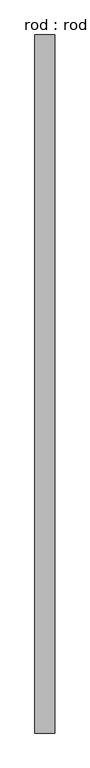
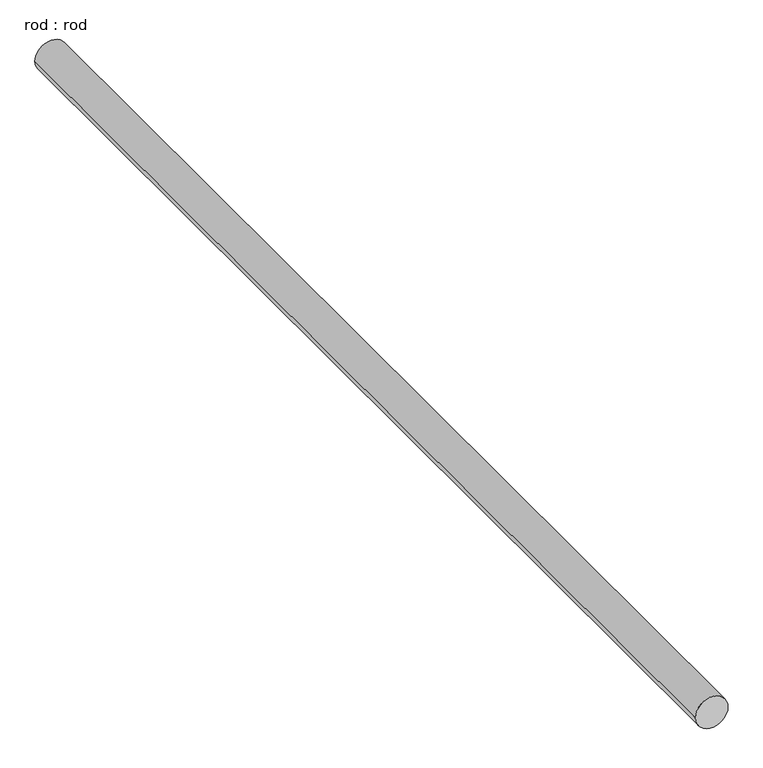
"""IFC4 building model written with IfcOpenShell, lengths in millimetres: proxy geometry, rod : rod."""

from ifc_helpers import new_model, si_unit, point, frame, frame_2d, origin, place, context, project, spatial, circle_curve, trimmed, segment, composite_curve, outline, extrude, source, transform, mapped, element, save


def rod_rod_52f87c7d(model_context):
    return source(origin(), model_context, "Body", "SweptSolid", [
        extrude(outline(composite_curve([segment(trimmed(circle_curve(frame_2d((0.0108462, 0.0)), 200.0), [point((0.0108462, 200.0))], [point((0.0108462, -200.0))], False, "CARTESIAN"), True, "CONTINUOUS"), segment(trimmed(circle_curve(frame_2d((0.0108462, 0.0)), 200.0), [point((0.0108462, -200.0))], [point((0.0108462, 200.0))], False, "CARTESIAN"), True, "CONTINUOUS")], self_intersect=False)), frame((0.0, -2925.1285275, 0.0), z_axis=(0.0, 1.0, 0.0), x_axis=(0.0, 0.0, 1.0)), (0.0, 0.0, 1.0), 14035.7142857),
    ])


if __name__ == "__main__":
    model = new_model("IFC4")
    model_context = context("Model", 3, world=origin())
    ifc_project = project(units=[si_unit("LENGTHUNIT", "METRE", prefix="MILLI")], contexts=[model_context])
    site = spatial("IfcSite", under=ifc_project)
    building = spatial("IfcBuilding", under=site)
    placement = place(None, origin())
    rod_rod_shape = rod_rod_52f87c7d(model_context)
    element("IfcBuildingElementProxy", 1, Name="rod : rod", ObjectType="rod : rod", at=placement, inside=building, context=model_context, shape_type="MappedRepresentation", body=[
        mapped(rod_rod_shape, transform((0.0, 0.0, 0.0), x_axis=(1.0, 0.0, 0.0), y_axis=(0.0, 1.0, 0.0), z_axis=(0.0, 0.0, 1.0))),
    ])
    save(model, "model.ifc")

# Revit data of these elements
# Type "rod : rod"
#   Default Elevation = 0
